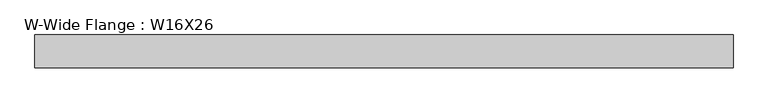
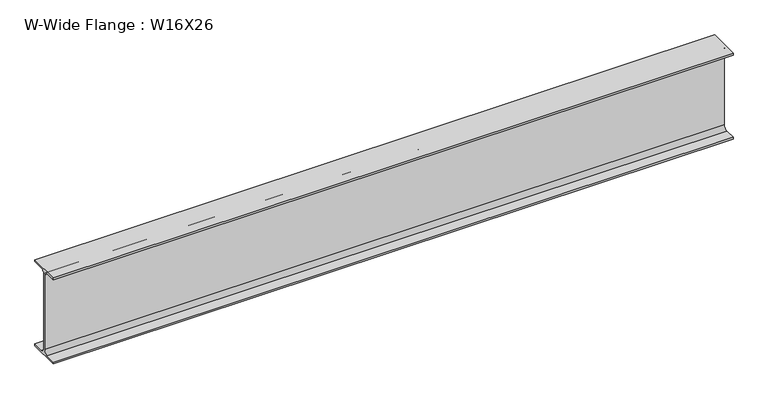
"""IFC4 building model written with IfcOpenShell, lengths in millimetres: beam geometry, W-Wide Flange : W16X26."""

from ifc_helpers import new_model, si_unit, point, frame, frame_2d, origin, place, context, project, spatial, polyline, circle_curve, trimmed, segment, composite_curve, outline, extrude, source, transform, mapped, element, save


def w_wide_flange_w16x26_c3b4808c(model_context):
    return source(origin(), model_context, "Body", "SweptSolid", [
        extrude(outline(composite_curve([segment(polyline([(69.85, -190.627), (69.85, -199.39), (-69.85, -199.39), (-69.85, -190.627), (-21.3995, -190.627)]), True, "CONTINUOUS"), segment(trimmed(circle_curve(frame_2d((-21.3995, -172.4025)), 18.2245), [point((-21.3995, -190.627))], [point((-3.175, -172.4025))], True, "CARTESIAN"), True, "CONTINUOUS"), segment(polyline([(-3.175, -172.4025), (-3.175, 172.4025)]), True, "CONTINUOUS"), segment(trimmed(circle_curve(frame_2d((-21.3995, 172.4025)), 18.2245), [point((-3.175, 172.4025))], [point((-21.3995, 190.627))], True, "CARTESIAN"), True, "CONTINUOUS"), segment(polyline([(-21.3995, 190.627), (-69.85, 190.627), (-69.85, 199.39), (69.85, 199.39), (69.85, 190.627), (21.3995, 190.627)]), True, "CONTINUOUS"), segment(trimmed(circle_curve(frame_2d((21.3995, 172.4025)), 18.2245), [point((21.3995, 190.627))], [point((3.175, 172.4025))], True, "CARTESIAN"), True, "CONTINUOUS"), segment(polyline([(3.175, 172.4025), (3.175, -172.4025)]), True, "CONTINUOUS"), segment(trimmed(circle_curve(frame_2d((21.3995, -172.4025)), 18.2245), [point((3.175, -172.4025))], [point((21.3995, -190.627))], True, "CARTESIAN"), True, "CONTINUOUS"), segment(polyline([(21.3995, -190.627), (69.85, -190.627)]), True, "CONTINUOUS")], self_intersect=False)), frame((-1498.6, 0.0, 0.0), z_axis=(1.0, 0.0, 0.0), x_axis=(0.0, 1.0, 0.0)), (0.0, 0.0, 1.0), 2978.15),
    ])


if __name__ == "__main__":
    model = new_model("IFC4")
    model_context = context("Model", 3, world=origin())
    ifc_project = project(units=[si_unit("LENGTHUNIT", "METRE", prefix="MILLI")], contexts=[model_context])
    site = spatial("IfcSite", under=ifc_project)
    building = spatial("IfcBuilding", under=site)
    placement = place(None, origin())
    w_wide_flange_w16x26_shape = w_wide_flange_w16x26_c3b4808c(model_context)
    element("IfcBeam", 1, ObjectType="W-Wide Flange : W16X26", at=placement, inside=building, context=model_context, shape_type="MappedRepresentation", body=[
        mapped(w_wide_flange_w16x26_shape, transform((0.0, 0.0, 0.0), x_axis=(1.0, 0.0, 0.0), y_axis=(0.0, 1.0, 0.0), z_axis=(0.0, 0.0, 1.0))),
    ])
    save(model, "model.ifc")

# Revit data of these elements
# Type "W-Wide Flange : W16X26"
#   Assembly Code = "B10"
#   W = 26
#   Length [instance default] = 5' - 0"
#   bf = 0' - 5 1/2"
#   d = 1' - 3.7"
#   k = 0' - 1 1/16"
#   k2 = 0' - 0.7175"
#   tf = 0' - 0.345"
#   tw = 0' - 0 1/4"
#   A = 0.0533333 SF
#   Structural Material [instance default] = Steel ASTM A992
# Element 1 (IfcBeam, "W-Wide Flange : W16X26")
#   Materials on its faces: "Steel ASTM A992"
# Materials
#   "Steel ASTM A992": class "Metal", colour RGB 199 199 199, transparency 0, Description = "Structural steel 50ksi", Cost = 0
